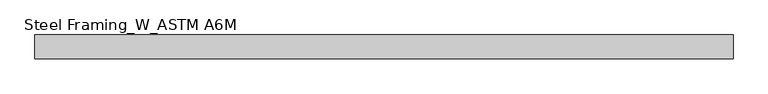
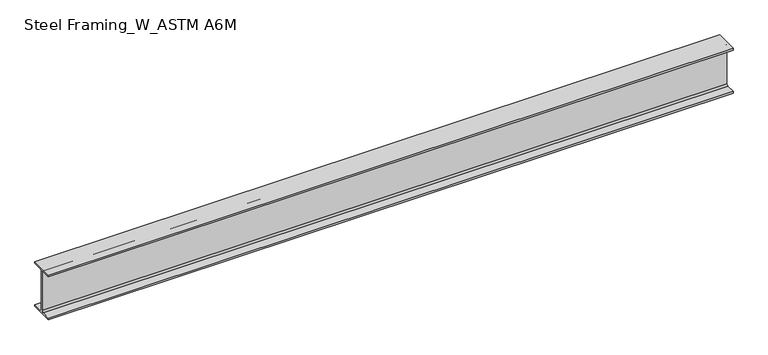
"""IFC4 building model written with IfcOpenShell, lengths in millimetres: beam geometry, Steel Framing_W_ASTM A6M : H_SB_AR_S02_W200x22.5_RB5."""

import ifcopenshell
import ifcopenshell.guid

model = None  # the IFC model being written
_history = None  # IfcOwnerHistory: only IFC2X3 demands one
_inside = {}  # id of a spatial element -> (the spatial element, [elements in it])
_under = {}  # id of a project, library or spatial element -> (it, [spatial elements below it])
_declared = {}  # id of a project -> (the project, [libraries it declares])
_typed = {}  # id of a type object -> (the type object, [elements of that type])
_made_of = {}  # id of a material, layer set ... -> (it, [elements and type objects made of it])


def new_model(schema):
    """Start an empty IFC model of exactly this schema.

    Asked for "IFC4X3", IfcOpenShell would pick the latest addendum, in which some entities
    have other attributes; the version numbers below select the first issue.
    IFC2X3 requires an IfcOwnerHistory on every rooted entity: one is made here for all.
    """
    global model, _history
    if schema == "IFC4X3":
        model = ifcopenshell.file(schema_version=(4, 3, 0, 0))
    else:
        model = ifcopenshell.file(schema=schema)
    _inside.clear()
    _under.clear()
    _declared.clear()
    _typed.clear()
    _made_of.clear()
    _history = None
    if model.schema == "IFC2X3":
        org = make("IfcOrganization", Name="unknown")
        user = make(
            "IfcPersonAndOrganization",
            ThePerson=make("IfcPerson", FamilyName="unknown"),
            TheOrganization=org,
        )
        app = make(
            "IfcApplication",
            ApplicationDeveloper=org,
            Version="unknown",
            ApplicationFullName="unknown",
            ApplicationIdentifier="unknown",
        )
        _history = make(
            "IfcOwnerHistory",
            OwningUser=user,
            OwningApplication=app,
            ChangeAction="ADDED",
            CreationDate=0,
        )
    return model


def make(cls, **values):
    """One entity of the class cls with the attributes given. An attribute that is None is left unset."""
    return model.create_entity(
        cls, **{name: value for name, value in values.items() if value is not None}
    )


def rooted(cls, **values):
    """An entity with a GlobalId (a new one), such as an element, a storey or a relation."""
    return make(cls, GlobalId=ifcopenshell.guid.new(), OwnerHistory=_history, **values)


def si_unit(unit_type, name, prefix=None):
    """IfcSIUnit, for example si_unit("LENGTHUNIT", "METRE", prefix="MILLI")."""
    return make("IfcSIUnit", UnitType=unit_type, Prefix=prefix, Name=name)


def assignment(units):
    """IfcUnitAssignment: the units of a project."""
    return None if units is None else make("IfcUnitAssignment", Units=units)


def point(xyz):
    """IfcCartesianPoint."""
    return None if xyz is None else make("IfcCartesianPoint", Coordinates=xyz)


def direction(xyz):
    """IfcDirection."""
    return None if xyz is None else make("IfcDirection", DirectionRatios=xyz)


def frame(location, z_axis=None, x_axis=None):
    """IfcAxis2Placement3D, a coordinate frame: its origin and axes. An axis left out is left unset."""
    return make(
        "IfcAxis2Placement3D",
        Location=point(location),
        Axis=direction(z_axis),
        RefDirection=direction(x_axis),
    )


def frame_2d(location, x_axis=None):
    """IfcAxis2Placement2D, a coordinate frame in the plane: its origin and x axis."""
    return make(
        "IfcAxis2Placement2D", Location=point(location), RefDirection=direction(x_axis)
    )


def origin():
    """The frame at (0, 0, 0) with its axes left unset."""
    return frame((0.0, 0.0, 0.0))


def place(relative_to, where):
    """IfcLocalPlacement: puts the frame where relative to a parent placement (None: the world)."""
    return make(
        "IfcLocalPlacement", PlacementRelTo=relative_to, RelativePlacement=where
    )


def context(
    kind, dimensions, precision=None, world=None, true_north=None, identifier=None
):
    """IfcGeometricRepresentationContext, for example the 3D "Model" context."""
    return make(
        "IfcGeometricRepresentationContext",
        ContextIdentifier=identifier,
        ContextType=kind,
        CoordinateSpaceDimension=dimensions,
        Precision=precision,
        WorldCoordinateSystem=world,
        TrueNorth=true_north,
    )


def project(units=None, contexts=None):
    """IfcProject with its units and contexts."""
    return rooted(
        "IfcProject",
        Name="project",
        RepresentationContexts=contexts,
        UnitsInContext=assignment(units),
    )


def spatial(cls, under=None, at=None, **own):
    """A site, building, storey or space (cls), placed at a placement, below another one or the project."""
    s = rooted(cls, ObjectPlacement=at, **own)
    if under is not None:
        _under.setdefault(under.id(), (under, []))[1].append(s)
    return s


def polyline(points):
    """IfcPolyline through the points."""
    return make("IfcPolyline", Points=[point(p) for p in points])


def circle_curve(where, radius):
    """IfcCircle in the frame where."""
    return make("IfcCircle", Position=where, Radius=radius)


def trimmed(basis, trim1, trim2, sense, master):
    """IfcTrimmedCurve: the piece of a basis curve between two trims."""
    return make(
        "IfcTrimmedCurve",
        BasisCurve=basis,
        Trim1=trim1,
        Trim2=trim2,
        SenseAgreement=sense,
        MasterRepresentation=master,
    )


def segment(curve, same_sense, transition):
    """IfcCompositeCurveSegment."""
    return make(
        "IfcCompositeCurveSegment",
        Transition=transition,
        SameSense=same_sense,
        ParentCurve=curve,
    )


def composite_curve(segments, self_intersect=None):
    """IfcCompositeCurve: segments joined end to end."""
    return make("IfcCompositeCurve", Segments=segments, SelfIntersect=self_intersect)


def outline(outer, holes=None, kind="AREA"):
    """IfcArbitraryClosedProfileDef: a profile drawn as a closed curve; with holes, ...WithVoids."""
    if holes is None:
        return make("IfcArbitraryClosedProfileDef", ProfileType=kind, OuterCurve=outer)
    return make(
        "IfcArbitraryProfileDefWithVoids",
        ProfileType=kind,
        OuterCurve=outer,
        InnerCurves=holes,
    )


def extrude(swept, where, along, depth):
    """IfcExtrudedAreaSolid: the profile swept, set in the frame where, extruded along a direction by depth."""
    return make(
        "IfcExtrudedAreaSolid",
        SweptArea=swept,
        Position=where,
        ExtrudedDirection=direction(along),
        Depth=depth,
    )


def shape(context_of_items, identifier, shape_type, items):
    """IfcShapeRepresentation: the items that make up one representation, for example the "Body"."""
    return make(
        "IfcShapeRepresentation",
        ContextOfItems=context_of_items,
        RepresentationIdentifier=identifier,
        RepresentationType=shape_type,
        Items=items,
    )


def source(mapping_origin, context_of_items, identifier, shape_type, items):
    """IfcRepresentationMap: a shape defined once, which mapped items show again and again."""
    return make(
        "IfcRepresentationMap",
        MappingOrigin=mapping_origin,
        MappedRepresentation=shape(context_of_items, identifier, shape_type, items),
    )


def transform(
    local_origin,
    x_axis=None,
    y_axis=None,
    z_axis=None,
    scale=None,
    scale2=None,
    scale3=None,
    uniform=True,
):
    """IfcCartesianTransformationOperator3D, or its non-uniform kind. x_axis, y_axis, z_axis: its Axis1, 2, 3."""
    if uniform:
        return make(
            "IfcCartesianTransformationOperator3D",
            Axis1=direction(x_axis),
            Axis2=direction(y_axis),
            LocalOrigin=point(local_origin),
            Scale=scale,
            Axis3=direction(z_axis),
        )
    return make(
        "IfcCartesianTransformationOperator3DnonUniform",
        Axis1=direction(x_axis),
        Axis2=direction(y_axis),
        LocalOrigin=point(local_origin),
        Scale=scale,
        Axis3=direction(z_axis),
        Scale2=scale2,
        Scale3=scale3,
    )


def mapped(mapping_source, mapping_target):
    """IfcMappedItem: shows the shape of a source again, moved by a transform."""
    return make(
        "IfcMappedItem", MappingSource=mapping_source, MappingTarget=mapping_target
    )


def made_of(thing, what):
    """Note that an element or type object is made of a material, layer set ...; save() writes the relation."""
    if what is not None:
        _made_of.setdefault(what.id(), (what, []))[1].append(thing)
    return thing


def element(
    cls,
    number,
    at=None,
    inside=None,
    cuts=None,
    type_object=None,
    material=None,
    context=None,
    identifier="Body",
    shape_type=None,
    held_by="IfcProductDefinitionShape",
    body=None,
    shapes=None,
    **own,
):
    """One element of the class cls, such as IfcWall. Its Tag is "e" and its number.

    at: its placement. inside: the storey or other place that contains it. cuts: it is an
    opening in that element (IfcRelVoidsElement). A single representation is given by context,
    identifier, shape_type and body (its items); several are given by shapes. held_by: the class
    of the entity that holds the representations. save() writes the other relations.
    """
    e = rooted(cls, Tag="e%d" % number, ObjectPlacement=at, **own)
    if body is not None:
        shapes = [shape(context, identifier, shape_type, body)]
    if shapes is not None:
        e.Representation = make(held_by, Representations=shapes)
    if inside is not None:
        _inside.setdefault(inside.id(), (inside, []))[1].append(e)
    if cuts is not None:
        rooted(
            "IfcRelVoidsElement", RelatingBuildingElement=cuts, RelatedOpeningElement=e
        )
    if type_object is not None:
        _typed.setdefault(type_object.id(), (type_object, []))[1].append(e)
    return made_of(e, material)


def aggregate(whole, parts):
    """IfcRelAggregates: a whole, such as a stair, and the parts it consists of."""
    return rooted("IfcRelAggregates", RelatingObject=whole, RelatedObjects=parts)


def save(model, path):
    """Write the relations noted so far, then the file.

    IfcRelAggregates (storeys below a building ...), IfcRelContainedInSpatialStructure (elements
    in a storey), IfcRelDefinesByType, IfcRelAssociatesMaterial and IfcRelDeclares: one each for
    every whole, place, type object, material and project.
    """
    for whole, parts in _under.values():
        aggregate(whole, parts)
    for where, things in _inside.values():
        rooted(
            "IfcRelContainedInSpatialStructure",
            RelatedElements=things,
            RelatingStructure=where,
        )
    for kind, things in _typed.values():
        rooted("IfcRelDefinesByType", RelatedObjects=things, RelatingType=kind)
    for what, things in _made_of.values():
        rooted("IfcRelAssociatesMaterial", RelatedObjects=things, RelatingMaterial=what)
    for by, libraries in _declared.values():
        rooted("IfcRelDeclares", RelatingContext=by, RelatedDefinitions=libraries)
    model.write(path)


def steel_framing_w_astm_a6m_c4277c11(model_context):
    return source(origin(), model_context, "Body", "SweptSolid", [
        extrude(outline(composite_curve([segment(polyline([(51.0, -95.0), (51.0, -103.0), (-51.0, -103.0), (-51.0, -95.0), (-10.71, -95.0)]), True, "CONTINUOUS"), segment(trimmed(circle_curve(frame_2d((-10.71, -87.4)), 7.6), [point((-10.71, -95.0))], [point((-3.11, -87.4))], True, "CARTESIAN"), True, "CONTINUOUS"), segment(polyline([(-3.11, -87.4), (-3.11, 87.4)]), True, "CONTINUOUS"), segment(trimmed(circle_curve(frame_2d((-10.71, 87.4)), 7.6), [point((-3.11, 87.4))], [point((-10.71, 95.0))], True, "CARTESIAN"), True, "CONTINUOUS"), segment(polyline([(-10.71, 95.0), (-51.0, 95.0), (-51.0, 103.0), (51.0, 103.0), (51.0, 95.0), (10.71, 95.0)]), True, "CONTINUOUS"), segment(trimmed(circle_curve(frame_2d((10.71, 87.4)), 7.6), [point((10.71, 95.0))], [point((3.11, 87.4))], True, "CARTESIAN"), True, "CONTINUOUS"), segment(polyline([(3.11, 87.4), (3.11, -87.4)]), True, "CONTINUOUS"), segment(trimmed(circle_curve(frame_2d((10.71, -87.4)), 7.6), [point((3.11, -87.4))], [point((10.71, -95.0))], True, "CARTESIAN"), True, "CONTINUOUS"), segment(polyline([(10.71, -95.0), (51.0, -95.0)]), True, "CONTINUOUS")], self_intersect=False)), frame((-1487.2, 0.0, 0.0), z_axis=(1.0, 0.0, 0.0), x_axis=(0.0, 1.0, 0.0)), (0.0, 0.0, 1.0), 2974.4),
    ])


if __name__ == "__main__":
    model = new_model("IFC4")
    model_context = context("Model", 3, world=origin())
    ifc_project = project(units=[si_unit("LENGTHUNIT", "METRE", prefix="MILLI")], contexts=[model_context])
    site = spatial("IfcSite", under=ifc_project)
    building = spatial("IfcBuilding", under=site)
    placement = place(None, origin())
    steel_framing_w_astm_a6m_shape = steel_framing_w_astm_a6m_c4277c11(model_context)
    element("IfcBeam", 1, ObjectType="Steel Framing_W_ASTM A6M : H_SB_AR_S02_W200x22.5_RB5", at=placement, inside=building, context=model_context, shape_type="MappedRepresentation", body=[
        mapped(steel_framing_w_astm_a6m_shape, transform((0.0, 0.0, 0.0), x_axis=(1.0, 0.0, 0.0), y_axis=(0.0, 1.0, 0.0), z_axis=(0.0, 0.0, 1.0))),
    ])
    save(model, "model.ifc")

# Revit data of these elements
# Type "Steel Framing_W_ASTM A6M : H_SB_AR_S02_W200x22.5_RB5"
#   Section Name Key = "W8x15"
#   Width = 10.2 cm
#   Web Thickness = 0.622 cm
#   Web Fillet = 0.76 cm
#   Warping Constant = 13900.0 cm⁶
#   Torsional Moment of Inertia = 5.70 cm⁴
#   Section Area = 28.6 cm²
#   Plastic Modulus weak axis = 43.8 cm³
#   Plastic Modulus strong axis = 223.0 cm³
#   Perimeter = 0.795 m²/m
#   Nominal Weight = 22.50 kgf/m
#   Moment of Inertia weak axis = 142.00 cm⁴
#   Moment of Inertia strong axis = 2000.00 cm⁴
#   Height = 20.6 cm
#   Flange Thickness = 0.8 cm
#   Elastic Modulus weak axis = 27.9 cm³
#   Elastic Modulus strong axis = 193.0 cm³
#   Centroid Vertical = 10.3 cm
#   Centroid Horizontal = 5.1 cm
#   Length [instance default] = 1500 mm
#   Structural Material [instance default] = Steel, 45-345
#   Bolt Spacing = 0
#   Assembly Code = ""
# Element 1 (IfcBeam, "Steel Framing_W_ASTM A6M : H_SB_AR_S02_W200x22.5_RB5")
#   Materials on its faces: "Steel, 45-345"
# Materials
#   "Steel, 45-345": class "Metal", colour RGB 189 187 185, transparency 0, Description = "Steel 345 MPa", Cost = 0
